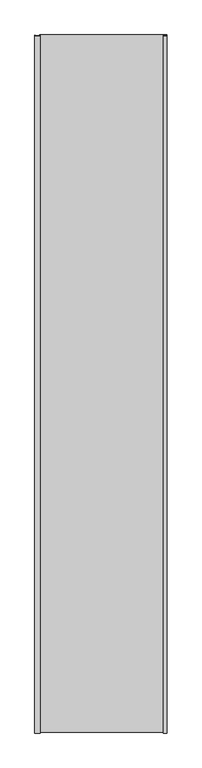
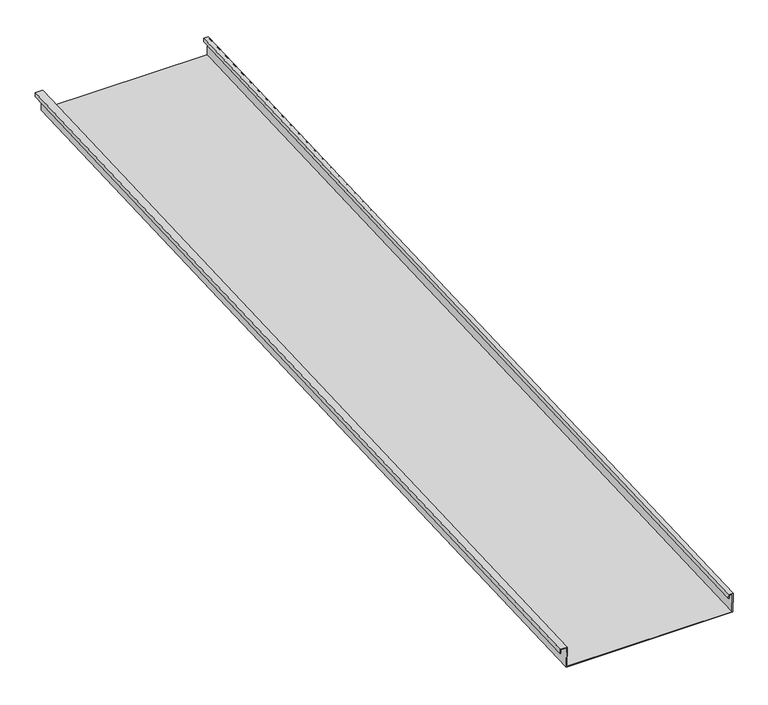
"""IFC4 building model written with IfcOpenShell, lengths in millimetres: proxy geometry, Generic Models 2:Generic Models 2:310765:Generic Models 2:310765 : Generic Models 2:Generic Models 2:310765:72 : Generic Models 2:Generic Models 2:310765:Generic Models 2:310765 : Generic Models 2:Generic Models 2:310765:300385."""

from ifc_helpers import new_model, si_unit, frame, origin, place, context, project, spatial, polyline, outline, extrude, source, transform, mapped, element, save


def generic_models_b364a00d(model_context):
    return source(origin(), model_context, "Body", "SweptSolid", [
        extrude(outline(polyline([(1.5875, 0.0), (1.5875, 50.8), (407.9875, 50.8), (407.9875, 1.5875), (396.875, 1.5875), (396.875, 11.1125), (398.4625, 11.1125), (398.4625, 3.175), (406.4, 3.175), (406.4, 49.2125), (3.175, 49.2125), (3.175, -1.5874999), (-14.2875, -1.5874999), (-14.2875, 9.525), (-12.7, 9.525), (-12.7, 0.0), (1.5875, 0.0)])), frame((667477.7263072, -581354.4345603, 3902.6697972), z_axis=(0.0, 0.9991330730923568, 0.041630544712067834), x_axis=(1.0, 0.0, 0.0)), (0.0, 0.0, 1.0), 2223.7764933),
    ])


if __name__ == "__main__":
    model = new_model("IFC4")
    model_context = context("Model", 3, world=origin())
    ifc_project = project(units=[si_unit("LENGTHUNIT", "METRE", prefix="MILLI")], contexts=[model_context])
    site = spatial("IfcSite", under=ifc_project)
    building = spatial("IfcBuilding", under=site)
    placement = place(None, origin())
    generic_models_shape = generic_models_b364a00d(model_context)
    element("IfcBuildingElementProxy", 1, Name="Generic Models 2:Generic Models 2:310765:Generic Models 2:310765 : Generic Models 2:Generic Models 2:310765:72 : Generic Models 2:Generic Models 2:310765:Generic Models 2:310765 : Generic Models 2:Generic Models 2:310765:300385", ObjectType="Generic Models 2:Generic Models 2:310765:Generic Models 2:310765 : Generic Models 2:Generic Models 2:310765:72 : Generic Models 2:Generic Models 2:310765:Generic Models 2:310765 : Generic Models 2:Generic Models 2:310765:300385", at=placement, inside=building, context=model_context, shape_type="MappedRepresentation", body=[
        mapped(generic_models_shape, transform((0.0, 0.0, 0.0), x_axis=(1.0, 0.0, 0.0), y_axis=(0.0, 1.0, 0.0), z_axis=(0.0, 0.0, 1.0))),
    ])
    save(model, "model.ifc")

# Revit data of these elements
# Type "Generic Models 2:Generic Models 2:310765:Generic Models 2:310765 : Generic Models 2:Generic Models 2:310765:72 : Generic Models 2:Generic Models 2:310765:Generic Models 2:310765 : Generic Models 2:Generic Models 2:310765:300385"
#   NameOverride = "Generic Models 2:Generic Models 2:310765:Generic Models 2:310765 : Generic Models 2:Generic Models 2:310765:300385"
#   ObjectTypeOverride = "Generic Models 2:310765 : Generic Models 2:Generic Models 2:310765"
#   Reference = "Generic Models 2"
#   Tag = "300385"
# Element 1 (IfcBuildingElementProxy, "Generic Models 2:Generic Models 2:310765:Generic Models 2:310765 : Generic Models 2:Generic Models 2:310765:72 : Generic Models 2:Generic Models 2:310765:Generic Models 2:310765 : Generic Models 2:Generic Models 2:310765:300385")
#   Materials on its faces: "THERMAL BROKEN ALUMINUM STOREFRONT FOR POLYCARBONATE"
# Materials
#   "THERMAL BROKEN ALUMINUM STOREFRONT FOR POLYCARBONATE": class "Unassigned", colour RGB 244 244 244, transparency 0, Keynote = "M07611300.01", Cost = 0
